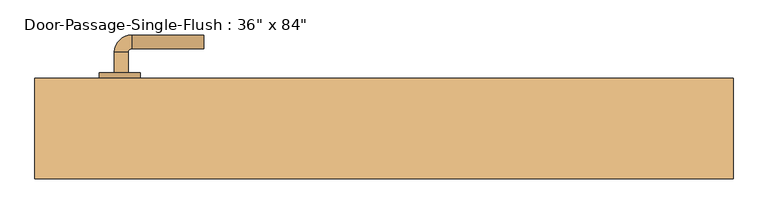
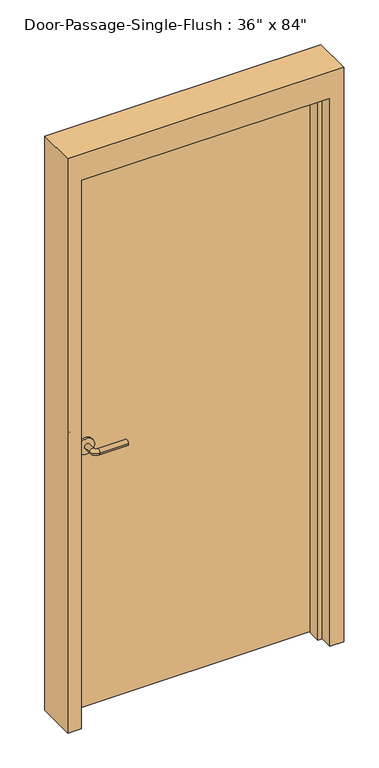
"""IFC4 building model written with IfcOpenShell, lengths in millimetres: door geometry."""

from ifc_helpers import new_model, si_unit, point, frame, frame_2d, origin, origin_with_axes, place, context, project, spatial, polyline, circle_curve, ellipse_curve, trimmed, segment, composite_curve, outline, extrude, faceted_brep, source, transform, mapped, element, save
from ifc_brep_helpers import plane_surface, cylinder_surface, revolved_surface, advanced_brep


def door_a376c32e(model_context):
    return source(origin(), model_context, "Body", "SolidModel", [
        advanced_brep(
        [(-392.190625, 30.1, 1016.0), (-372.190625, 30.1, 1016.0), (-372.190625, 0.1, 1016.0), (-392.190625, 0.1, 1016.0), (-367.190625, -4.9, 1016.0), (-367.190625, -24.9, 1016.0), (-262.190625, -24.9, 1016.0), (-262.190625, -4.9, 1016.0)],
        [
            (0, 1, circle_curve(frame((-382.190625, 30.1, 1016.0), z_axis=(0.0, 1.0, 0.0), x_axis=(1.0, 0.0, 0.0)), 10.0)),
            (1, 0, circle_curve(frame((-382.190625, 30.1, 1016.0), z_axis=(0.0, 1.0, 0.0), x_axis=(1.0, 0.0, 0.0)), 10.0)),
            (1, 2),
            (2, 3, circle_curve(frame((-382.190625, 0.1, 1016.0), z_axis=(0.0, 1.0, 0.0), x_axis=(1.0, 0.0, 0.0)), 10.0)),
            (3, 0),
            (3, 2, circle_curve(frame((-382.190625, 0.1, 1016.0), z_axis=(0.0, 1.0, 0.0), x_axis=(1.0, 0.0, 0.0)), 10.0)),
            (4, 5, circle_curve(frame((-367.190625, -14.9, 1016.0), z_axis=(-1.0, 0.0, 0.0), x_axis=(0.0, 1.0, 0.0)), 10.0)),
            (5, 3, circle_curve(frame((-367.190625, 0.1, 1016.0), z_axis=(0.0, 0.0, -1.0), x_axis=(-1.0, 0.0, 0.0)), 25.0)),
            (2, 4, circle_curve(frame((-367.190625, 0.1, 1016.0), z_axis=(0.0, 0.0, 1.0), x_axis=(-1.0, 0.0, 0.0)), 5.0)),
            (5, 4, circle_curve(frame((-367.190625, -14.9, 1016.0), z_axis=(-1.0, 0.0, 0.0), x_axis=(0.0, 1.0, 0.0)), 10.0)),
            (6, 7, circle_curve(frame((-262.190625, -14.9, 1016.0), z_axis=(1.0, 0.0, 0.0), x_axis=(0.0, 1.0, 0.0)), 10.0)),
            (7, 6, circle_curve(frame((-262.190625, -14.9, 1016.0), z_axis=(1.0, 0.0, 0.0), x_axis=(0.0, 1.0, 0.0)), 10.0)),
            (4, 7),
            (6, 5),
        ],
        [
            plane_surface(frame((-382.190625, 30.1, 1016.0), z_axis=(0.0, 1.0, 0.0), x_axis=(0.0, 0.0, 1.0))),
            cylinder_surface(frame((-382.190625, 30.1, 1016.0), z_axis=(0.0, 1.0, 0.0), x_axis=(1.0, 0.0, 0.0)), 10.0),
            revolved_surface(trimmed(ellipse_curve(frame((-382.190625, 0.1, 1016.0), z_axis=(0.0, -1.0, 0.0), x_axis=(1.0, 0.0, 0.0)), 10.0, 10.0), [point((-392.190625, 0.1, 1016.0))], [point((-372.190625, 0.1, 1016.0))], True, "CARTESIAN"), (-367.190625, 0.1, 1016.0), (0.0, 0.0, -1.0)),
            revolved_surface(trimmed(ellipse_curve(frame((-382.190625, 0.1, 1016.0), z_axis=(0.0, -1.0, 0.0), x_axis=(1.0, 0.0, 0.0)), 10.0, 10.0), [point((-372.190625, 0.1, 1016.0))], [point((-392.190625, 0.1, 1016.0))], True, "CARTESIAN"), (-367.190625, 0.1, 1016.0), (0.0, 0.0, -1.0)),
            plane_surface(frame((-262.190625, -14.9, 1016.0), z_axis=(1.0, 0.0, 0.0), x_axis=(0.0, 0.0, 1.0))),
            cylinder_surface(frame((-367.190625, -14.9, 1016.0), z_axis=(-1.0, 0.0, 0.0), x_axis=(0.0, 1.0, 0.0)), 10.0),
        ],
        [
            (0, [[1, 2]]),
            (1, [[3, 4, 5, -2]]),
            (1, [[-5, 6, -3, -1]]),
            (2, [[7, 8, -4, 9]]),
            (3, [[10, -9, -6, -8]]),
            (4, [[11, 12]]),
            (5, [[13, -11, 14, -7]]),
            (5, [[-14, -12, -13, -10]]),
        ],
    ),
        extrude(outline(composite_curve([segment(trimmed(circle_curve(frame_2d((1016.0, -384.690625)), 30.0), [point((1016.0, -414.690625))], [point((1016.0, -354.690625))], False, "CARTESIAN"), True, "CONTINUOUS"), segment(trimmed(circle_curve(frame_2d((1016.0, -384.690625)), 30.0), [point((1016.0, -354.690625))], [point((1016.0, -414.690625))], False, "CARTESIAN"), True, "CONTINUOUS")], self_intersect=False)), frame((0.0, 30.1, 0.0), z_axis=(0.0, 1.0, 0.0), x_axis=(0.0, 0.0, 1.0)), (0.0, 0.0, 1.0), 8.0),
        advanced_brep(
        [(-392.190625, 90.55, 1016.0), (-372.190625, 90.55, 1016.0), (-392.190625, 120.55, 1016.0), (-372.190625, 120.55, 1016.0), (-367.190625, 125.55, 1016.0), (-367.190625, 145.55, 1016.0), (-262.190625, 145.55, 1016.0), (-262.190625, 125.55, 1016.0)],
        [
            (0, 1, circle_curve(frame((-382.190625, 90.55, 1016.0), z_axis=(0.0, -1.0, 0.0), x_axis=(1.0, 0.0, 0.0)), 10.0)),
            (1, 0, circle_curve(frame((-382.190625, 90.55, 1016.0), z_axis=(0.0, -1.0, 0.0), x_axis=(1.0, 0.0, 0.0)), 10.0)),
            (0, 2),
            (2, 3, circle_curve(frame((-382.190625, 120.55, 1016.0), z_axis=(0.0, -1.0, 0.0), x_axis=(1.0, 0.0, 0.0)), 10.0)),
            (3, 1),
            (3, 2, circle_curve(frame((-382.190625, 120.55, 1016.0), z_axis=(0.0, -1.0, 0.0), x_axis=(1.0, 0.0, 0.0)), 10.0)),
            (4, 3, circle_curve(frame((-367.190625, 120.55, 1016.0), z_axis=(0.0, 0.0, 1.0), x_axis=(-1.0, 0.0, 0.0)), 5.0)),
            (2, 5, circle_curve(frame((-367.190625, 120.55, 1016.0), z_axis=(0.0, 0.0, -1.0), x_axis=(-1.0, 0.0, 0.0)), 25.0)),
            (5, 4, circle_curve(frame((-367.190625, 135.55, 1016.0), z_axis=(-1.0, 0.0, 0.0), x_axis=(0.0, -1.0, 0.0)), 10.0)),
            (4, 5, circle_curve(frame((-367.190625, 135.55, 1016.0), z_axis=(-1.0, 0.0, 0.0), x_axis=(0.0, -1.0, 0.0)), 10.0)),
            (6, 7, circle_curve(frame((-262.190625, 135.55, 1016.0), z_axis=(1.0, 0.0, 0.0), x_axis=(0.0, -1.0, 0.0)), 10.0)),
            (7, 6, circle_curve(frame((-262.190625, 135.55, 1016.0), z_axis=(1.0, 0.0, 0.0), x_axis=(0.0, -1.0, 0.0)), 10.0)),
            (5, 6),
            (7, 4),
        ],
        [
            plane_surface(frame((-382.190625, 90.55, 1016.0), z_axis=(0.0, -1.0, 0.0), x_axis=(0.0, 0.0, 1.0))),
            cylinder_surface(frame((-382.190625, 90.55, 1016.0), z_axis=(0.0, -1.0, 0.0), x_axis=(1.0, 0.0, 0.0)), 10.0),
            revolved_surface(trimmed(ellipse_curve(frame((-382.190625, 120.55, 1016.0), z_axis=(0.0, -1.0, 0.0), x_axis=(1.0, 0.0, 0.0)), 10.0, 10.0), [point((-392.190625, 120.55, 1016.0))], [point((-372.190625, 120.55, 1016.0))], True, "CARTESIAN"), (-367.190625, 120.55, 1016.0), (0.0, 0.0, -1.0)),
            revolved_surface(trimmed(ellipse_curve(frame((-382.190625, 120.55, 1016.0), z_axis=(0.0, -1.0, 0.0), x_axis=(1.0, 0.0, 0.0)), 10.0, 10.0), [point((-372.190625, 120.55, 1016.0))], [point((-392.190625, 120.55, 1016.0))], True, "CARTESIAN"), (-367.190625, 120.55, 1016.0), (0.0, 0.0, -1.0)),
            plane_surface(frame((-262.190625, 135.55, 1016.0), z_axis=(1.0, 0.0, 0.0), x_axis=(0.0, 0.0, 1.0))),
            cylinder_surface(frame((-367.190625, 135.55, 1016.0), z_axis=(-1.0, 0.0, 0.0), x_axis=(0.0, -1.0, 0.0)), 10.0),
        ],
        [
            (0, [[1, 2]]),
            (1, [[-1, 3, 4, 5]]),
            (1, [[-2, -5, 6, -3]]),
            (2, [[7, -4, 8, 9]]),
            (3, [[-8, -6, -7, 10]]),
            (4, [[11, 12]]),
            (5, [[-9, 13, -12, 14]]),
            (5, [[-10, -14, -11, -13]]),
        ],
    ),
        extrude(outline(composite_curve([segment(trimmed(circle_curve(frame_2d((1016.0, -384.690625)), 30.0), [point((1016.0, -414.690625))], [point((1016.0, -354.690625))], False, "CARTESIAN"), True, "CONTINUOUS"), segment(trimmed(circle_curve(frame_2d((1016.0, -384.690625)), 30.0), [point((1016.0, -354.690625))], [point((1016.0, -414.690625))], False, "CARTESIAN"), True, "CONTINUOUS")], self_intersect=False)), frame((0.0, 82.55, 0.0), z_axis=(0.0, 1.0, 0.0), x_axis=(0.0, 0.0, 1.0)), (0.0, 0.0, 1.0), 8.0),
        faceted_brep([(457.2, 33.3375, 0.0), (457.2, 82.55, 0.0), (508.0, 82.55, 0.0), (508.0, -63.5, 0.0), (457.2, -63.5, 0.0), (457.2, -14.2875, 0.0), (441.325, -14.2875, 0.0), (441.325, 33.3375, 0.0), (457.2, 33.3375, 2133.6), (457.2, 82.55, 2133.6), (-457.2, 82.55, 2133.6), (-457.2, 82.55, 0.0), (-508.0, 82.55, 0.0), (-508.0, 82.55, 2235.2), (508.0, 82.55, 2235.2), (508.0, -63.5, 2235.2), (-508.0, -63.5, 2235.2), (-508.0, -63.5, 0.0), (-457.2, -63.5, 0.0), (-457.2, -63.5, 2133.6), (457.2, -63.5, 2133.6), (457.2, -14.2875, 2133.6), (-457.2, -14.2875, 2133.6), (-457.2, -14.2875, 0.0), (-441.325, -14.2875, 0.0), (-441.325, -14.2875, 2117.725), (441.325, -14.2875, 2117.725), (441.325, 33.3375, 2117.725), (-441.325, 33.3375, 2117.725), (-441.325, 33.3375, 0.0), (-457.2, 33.3375, 0.0), (-457.2, 33.3375, 2133.6)], [[[0, 1, 2, 3, 4, 5, 6, 7]], [[1, 0, 8, 9]], [[2, 1, 9, 10, 11, 12, 13, 14]], [[3, 2, 14, 15]], [[4, 3, 15, 16, 17, 18, 19, 20]], [[5, 4, 20, 21]], [[6, 5, 21, 22, 23, 24, 25, 26]], [[7, 6, 26, 27]], [[0, 7, 27, 28, 29, 30, 31, 8]], [[9, 8, 31, 10]], [[20, 19, 22, 21]], [[26, 25, 28, 27]], [[12, 11, 30, 29, 24, 23, 18, 17]], [[11, 10, 31, 30]], [[13, 12, 17, 16]], [[19, 18, 23, 22]], [[25, 24, 29, 28]], [[15, 14, 13, 16]]]),
        extrude(outline(polyline([(457.2, 38.1), (-457.2, 38.1), (-457.2, 82.55), (457.2, 82.55), (457.2, 38.1)])), origin_with_axes(), (0.0, 0.0, 1.0), 2133.6),
    ])


if __name__ == "__main__":
    model = new_model("IFC4")
    model_context = context("Model", 3, world=origin())
    ifc_project = project(units=[si_unit("LENGTHUNIT", "METRE", prefix="MILLI")], contexts=[model_context])
    site = spatial("IfcSite", under=ifc_project)
    building = spatial("IfcBuilding", under=site)
    placement = place(None, origin())
    door_shape = door_a376c32e(model_context)
    element("IfcDoor", 1, ObjectType="Door-Passage-Single-Flush : 36\" x 84\"", at=placement, inside=building, context=model_context, shape_type="MappedRepresentation", body=[
        mapped(door_shape, transform((0.0, 0.0, 0.0), x_axis=(1.0, 0.0, 0.0), y_axis=(0.0, 1.0, 0.0), z_axis=(0.0, 0.0, 1.0))),
    ])
    save(model, "model.ifc")

# Revit data of these elements
# Type "Door-Passage-Single-Flush : 36\" x 84\""
#   Type Mark = "1"
#   Assembly Code = "B2030200"
#   Analytic Construction = "Wooden"
#   Thickness = 0' - 1 3/4"
#   Thermal Resistance (R) = 2.5876 (h·ft²·°F)/BTU
#   Swing Angle [instance default] = 90.00°
#   Strike Height = 3' - 4"
#   Rough Width [instance default] = 3' - 4"
#   Rough Height [instance default] = 7' - 4"
#   MF Opening Height [instance default] = 0' - 4"
#   MF Opening Width [instance default] = 0' - 4"
#   Inset Calculate [instance default] = 0' - 4"
#   Masonry Inset [instance default] = 0' - 1"
#   Height = 7' - 0"
#   Width = 3' - 0"
#   Heat Transfer Coefficient (U) = 0.3865 BTU/(h·ft²·°F)
#   Masonry Frame Depth = 0' - 5 3/4"
#   Function = 0
#   Masonry Frame [instance default] = yes
#   Function = 1
#   Dry Wall Frame [instance default] = no
#   Panel Material = Wood - Birch
#   Frame Material = Metal - Paint Finish - Grey
#   Door Handle Material = Aluminum
#   Visual Light Transmittance = 0
#   Solar Heat Gain Coefficient = 0
#   Wall Closure = (empty or 0)
# Element 1 (IfcDoor, "Door-Passage-Single-Flush : 36\" x 84\"")
#   Materials on its faces: "Aluminum", "Metal - Paint Finish - Grey", "Wood - Birch"
# Materials
#   "Wood - Birch": class "Unassigned", colour RGB 224 178 126, transparency 0
#   "Metal - Paint Finish - Grey": class "Paint", colour RGB 104 104 104, transparency 0, Cost = 0
#   "Aluminum": class "Metal", colour RGB 120 120 120, transparency 0, Description = "Aluminum 6061", Cost = 0
